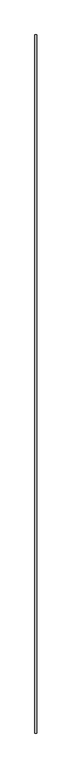
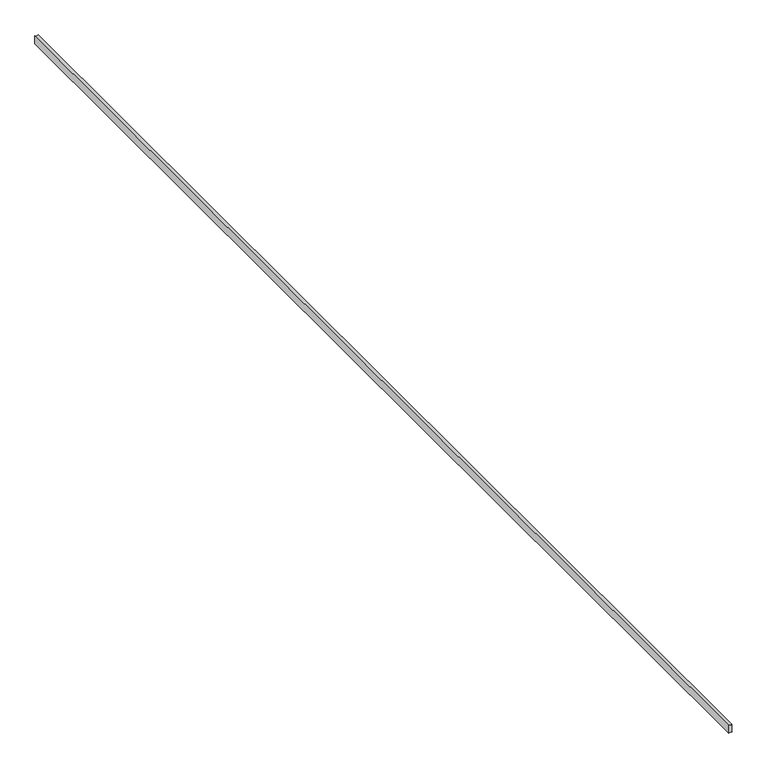
"""IFC4 building model written with IfcOpenShell, lengths in millimetres: proxy geometry, Joint043 17085 : Joint043 17085."""

import ifcopenshell
import ifcopenshell.guid

model = None  # the IFC model being written
_history = None  # IfcOwnerHistory: only IFC2X3 demands one
_inside = {}  # id of a spatial element -> (the spatial element, [elements in it])
_under = {}  # id of a project, library or spatial element -> (it, [spatial elements below it])
_declared = {}  # id of a project -> (the project, [libraries it declares])
_typed = {}  # id of a type object -> (the type object, [elements of that type])
_made_of = {}  # id of a material, layer set ... -> (it, [elements and type objects made of it])


def new_model(schema):
    """Start an empty IFC model of exactly this schema.

    Asked for "IFC4X3", IfcOpenShell would pick the latest addendum, in which some entities
    have other attributes; the version numbers below select the first issue.
    IFC2X3 requires an IfcOwnerHistory on every rooted entity: one is made here for all.
    """
    global model, _history
    if schema == "IFC4X3":
        model = ifcopenshell.file(schema_version=(4, 3, 0, 0))
    else:
        model = ifcopenshell.file(schema=schema)
    _inside.clear()
    _under.clear()
    _declared.clear()
    _typed.clear()
    _made_of.clear()
    _history = None
    if model.schema == "IFC2X3":
        org = make("IfcOrganization", Name="unknown")
        user = make(
            "IfcPersonAndOrganization",
            ThePerson=make("IfcPerson", FamilyName="unknown"),
            TheOrganization=org,
        )
        app = make(
            "IfcApplication",
            ApplicationDeveloper=org,
            Version="unknown",
            ApplicationFullName="unknown",
            ApplicationIdentifier="unknown",
        )
        _history = make(
            "IfcOwnerHistory",
            OwningUser=user,
            OwningApplication=app,
            ChangeAction="ADDED",
            CreationDate=0,
        )
    return model


def make(cls, **values):
    """One entity of the class cls with the attributes given. An attribute that is None is left unset."""
    return model.create_entity(
        cls, **{name: value for name, value in values.items() if value is not None}
    )


def rooted(cls, **values):
    """An entity with a GlobalId (a new one), such as an element, a storey or a relation."""
    return make(cls, GlobalId=ifcopenshell.guid.new(), OwnerHistory=_history, **values)


def si_unit(unit_type, name, prefix=None):
    """IfcSIUnit, for example si_unit("LENGTHUNIT", "METRE", prefix="MILLI")."""
    return make("IfcSIUnit", UnitType=unit_type, Prefix=prefix, Name=name)


def assignment(units):
    """IfcUnitAssignment: the units of a project."""
    return None if units is None else make("IfcUnitAssignment", Units=units)


def point(xyz):
    """IfcCartesianPoint."""
    return None if xyz is None else make("IfcCartesianPoint", Coordinates=xyz)


def direction(xyz):
    """IfcDirection."""
    return None if xyz is None else make("IfcDirection", DirectionRatios=xyz)


def frame(location, z_axis=None, x_axis=None):
    """IfcAxis2Placement3D, a coordinate frame: its origin and axes. An axis left out is left unset."""
    return make(
        "IfcAxis2Placement3D",
        Location=point(location),
        Axis=direction(z_axis),
        RefDirection=direction(x_axis),
    )


def frame_2d(location, x_axis=None):
    """IfcAxis2Placement2D, a coordinate frame in the plane: its origin and x axis."""
    return make(
        "IfcAxis2Placement2D", Location=point(location), RefDirection=direction(x_axis)
    )


def origin():
    """The frame at (0, 0, 0) with its axes left unset."""
    return frame((0.0, 0.0, 0.0))


def place(relative_to, where):
    """IfcLocalPlacement: puts the frame where relative to a parent placement (None: the world)."""
    return make(
        "IfcLocalPlacement", PlacementRelTo=relative_to, RelativePlacement=where
    )


def context(
    kind, dimensions, precision=None, world=None, true_north=None, identifier=None
):
    """IfcGeometricRepresentationContext, for example the 3D "Model" context."""
    return make(
        "IfcGeometricRepresentationContext",
        ContextIdentifier=identifier,
        ContextType=kind,
        CoordinateSpaceDimension=dimensions,
        Precision=precision,
        WorldCoordinateSystem=world,
        TrueNorth=true_north,
    )


def project(units=None, contexts=None):
    """IfcProject with its units and contexts."""
    return rooted(
        "IfcProject",
        Name="project",
        RepresentationContexts=contexts,
        UnitsInContext=assignment(units),
    )


def spatial(cls, under=None, at=None, **own):
    """A site, building, storey or space (cls), placed at a placement, below another one or the project."""
    s = rooted(cls, ObjectPlacement=at, **own)
    if under is not None:
        _under.setdefault(under.id(), (under, []))[1].append(s)
    return s


def polyline(points):
    """IfcPolyline through the points."""
    return make("IfcPolyline", Points=[point(p) for p in points])


def circle_curve(where, radius):
    """IfcCircle in the frame where."""
    return make("IfcCircle", Position=where, Radius=radius)


def trimmed(basis, trim1, trim2, sense, master):
    """IfcTrimmedCurve: the piece of a basis curve between two trims."""
    return make(
        "IfcTrimmedCurve",
        BasisCurve=basis,
        Trim1=trim1,
        Trim2=trim2,
        SenseAgreement=sense,
        MasterRepresentation=master,
    )


def segment(curve, same_sense, transition):
    """IfcCompositeCurveSegment."""
    return make(
        "IfcCompositeCurveSegment",
        Transition=transition,
        SameSense=same_sense,
        ParentCurve=curve,
    )


def composite_curve(segments, self_intersect=None):
    """IfcCompositeCurve: segments joined end to end."""
    return make("IfcCompositeCurve", Segments=segments, SelfIntersect=self_intersect)


def outline(outer, holes=None, kind="AREA"):
    """IfcArbitraryClosedProfileDef: a profile drawn as a closed curve; with holes, ...WithVoids."""
    if holes is None:
        return make("IfcArbitraryClosedProfileDef", ProfileType=kind, OuterCurve=outer)
    return make(
        "IfcArbitraryProfileDefWithVoids",
        ProfileType=kind,
        OuterCurve=outer,
        InnerCurves=holes,
    )


def extrude(swept, where, along, depth):
    """IfcExtrudedAreaSolid: the profile swept, set in the frame where, extruded along a direction by depth."""
    return make(
        "IfcExtrudedAreaSolid",
        SweptArea=swept,
        Position=where,
        ExtrudedDirection=direction(along),
        Depth=depth,
    )


def shape(context_of_items, identifier, shape_type, items):
    """IfcShapeRepresentation: the items that make up one representation, for example the "Body"."""
    return make(
        "IfcShapeRepresentation",
        ContextOfItems=context_of_items,
        RepresentationIdentifier=identifier,
        RepresentationType=shape_type,
        Items=items,
    )


def source(mapping_origin, context_of_items, identifier, shape_type, items):
    """IfcRepresentationMap: a shape defined once, which mapped items show again and again."""
    return make(
        "IfcRepresentationMap",
        MappingOrigin=mapping_origin,
        MappedRepresentation=shape(context_of_items, identifier, shape_type, items),
    )


def transform(
    local_origin,
    x_axis=None,
    y_axis=None,
    z_axis=None,
    scale=None,
    scale2=None,
    scale3=None,
    uniform=True,
):
    """IfcCartesianTransformationOperator3D, or its non-uniform kind. x_axis, y_axis, z_axis: its Axis1, 2, 3."""
    if uniform:
        return make(
            "IfcCartesianTransformationOperator3D",
            Axis1=direction(x_axis),
            Axis2=direction(y_axis),
            LocalOrigin=point(local_origin),
            Scale=scale,
            Axis3=direction(z_axis),
        )
    return make(
        "IfcCartesianTransformationOperator3DnonUniform",
        Axis1=direction(x_axis),
        Axis2=direction(y_axis),
        LocalOrigin=point(local_origin),
        Scale=scale,
        Axis3=direction(z_axis),
        Scale2=scale2,
        Scale3=scale3,
    )


def mapped(mapping_source, mapping_target):
    """IfcMappedItem: shows the shape of a source again, moved by a transform."""
    return make(
        "IfcMappedItem", MappingSource=mapping_source, MappingTarget=mapping_target
    )


def made_of(thing, what):
    """Note that an element or type object is made of a material, layer set ...; save() writes the relation."""
    if what is not None:
        _made_of.setdefault(what.id(), (what, []))[1].append(thing)
    return thing


def element(
    cls,
    number,
    at=None,
    inside=None,
    cuts=None,
    type_object=None,
    material=None,
    context=None,
    identifier="Body",
    shape_type=None,
    held_by="IfcProductDefinitionShape",
    body=None,
    shapes=None,
    **own,
):
    """One element of the class cls, such as IfcWall. Its Tag is "e" and its number.

    at: its placement. inside: the storey or other place that contains it. cuts: it is an
    opening in that element (IfcRelVoidsElement). A single representation is given by context,
    identifier, shape_type and body (its items); several are given by shapes. held_by: the class
    of the entity that holds the representations. save() writes the other relations.
    """
    e = rooted(cls, Tag="e%d" % number, ObjectPlacement=at, **own)
    if body is not None:
        shapes = [shape(context, identifier, shape_type, body)]
    if shapes is not None:
        e.Representation = make(held_by, Representations=shapes)
    if inside is not None:
        _inside.setdefault(inside.id(), (inside, []))[1].append(e)
    if cuts is not None:
        rooted(
            "IfcRelVoidsElement", RelatingBuildingElement=cuts, RelatedOpeningElement=e
        )
    if type_object is not None:
        _typed.setdefault(type_object.id(), (type_object, []))[1].append(e)
    return made_of(e, material)


def aggregate(whole, parts):
    """IfcRelAggregates: a whole, such as a stair, and the parts it consists of."""
    return rooted("IfcRelAggregates", RelatingObject=whole, RelatedObjects=parts)


def save(model, path):
    """Write the relations noted so far, then the file.

    IfcRelAggregates (storeys below a building ...), IfcRelContainedInSpatialStructure (elements
    in a storey), IfcRelDefinesByType, IfcRelAssociatesMaterial and IfcRelDeclares: one each for
    every whole, place, type object, material and project.
    """
    for whole, parts in _under.values():
        aggregate(whole, parts)
    for where, things in _inside.values():
        rooted(
            "IfcRelContainedInSpatialStructure",
            RelatedElements=things,
            RelatingStructure=where,
        )
    for kind, things in _typed.values():
        rooted("IfcRelDefinesByType", RelatedObjects=things, RelatingType=kind)
    for what, things in _made_of.values():
        rooted("IfcRelAssociatesMaterial", RelatedObjects=things, RelatingMaterial=what)
    for by, libraries in _declared.values():
        rooted("IfcRelDeclares", RelatingContext=by, RelatedDefinitions=libraries)
    model.write(path)


def generic_models_89c7964b(model_context):
    return source(origin(), model_context, "Body", "SweptSolid", [
        extrude(outline(composite_curve([segment(polyline([(36707.8109404, 6041.1562997), (36721.7109375, 6041.1562997)]), True, "CONTINUOUS"), segment(trimmed(circle_curve(frame_2d((36725.0040268, 6038.4523044)), 4.260989), [point((36721.7109375, 6041.1562997))], [point((36721.7109375, 6035.7483091))], True, "CARTESIAN"), True, "CONTINUOUS"), segment(polyline([(36721.7109375, 6035.7483091), (36707.9131594, 6035.7483091)]), True, "CONTINUOUS"), segment(trimmed(circle_curve(frame_2d((36704.7568736, 6038.393612)), 4.1182239), [point((36707.9131594, 6035.7483091))], [point((36707.8109404, 6041.1562997))], True, "CARTESIAN"), True, "CONTINUOUS")], self_intersect=False)), frame((0.0, 2217.3609973, 0.0), z_axis=(0.0, 1.0, 0.0), x_axis=(0.0, 0.0, 1.0)), (0.0, 0.0, 1.0), 2000.0),
    ])


if __name__ == "__main__":
    model = new_model("IFC4")
    model_context = context("Model", 3, world=origin())
    ifc_project = project(units=[si_unit("LENGTHUNIT", "METRE", prefix="MILLI")], contexts=[model_context])
    site = spatial("IfcSite", under=ifc_project)
    building = spatial("IfcBuilding", under=site)
    placement = place(None, origin())
    generic_models_shape = generic_models_89c7964b(model_context)
    element("IfcBuildingElementProxy", 1, Name="Joint043 17085 : Joint043 17085", ObjectType="Joint043 17085 : Joint043 17085", at=placement, inside=building, context=model_context, shape_type="MappedRepresentation", body=[
        mapped(generic_models_shape, transform((0.0, 0.0, 0.0), x_axis=(1.0, 0.0, 0.0), y_axis=(0.0, 1.0, 0.0), z_axis=(0.0, 0.0, 1.0))),
    ])
    save(model, "model.ifc")

# Revit data of these elements
# Type "Joint043 17085 : Joint043 17085"
#   NameOverride = "Joint043"
# Element 1 (IfcBuildingElementProxy, "Joint043 17085 : Joint043 17085")
#   Materials on its faces: "SEALANT"
# Materials
#   "SEALANT": class "Unassigned", colour RGB 142 225 148, transparency 0
